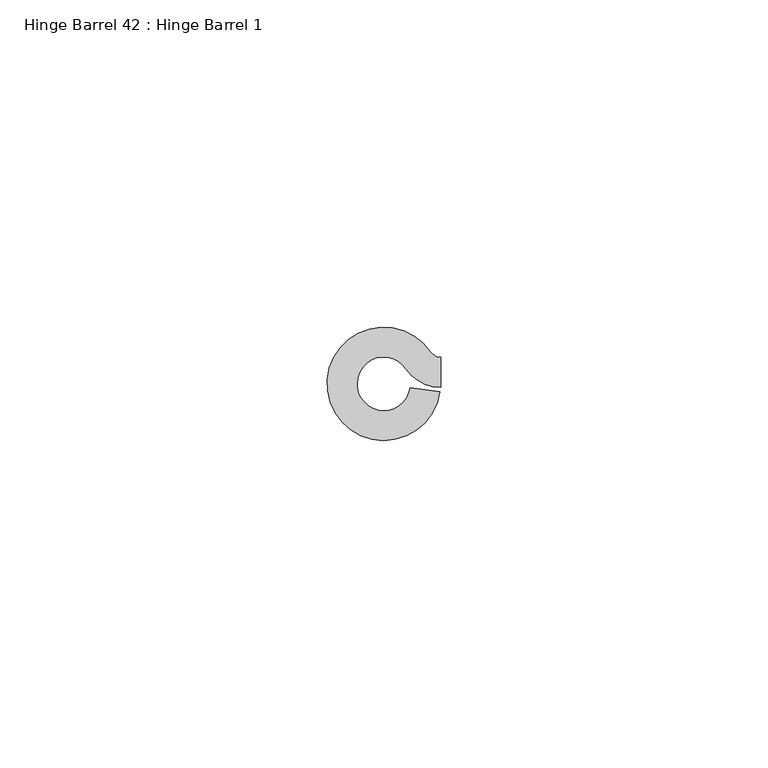
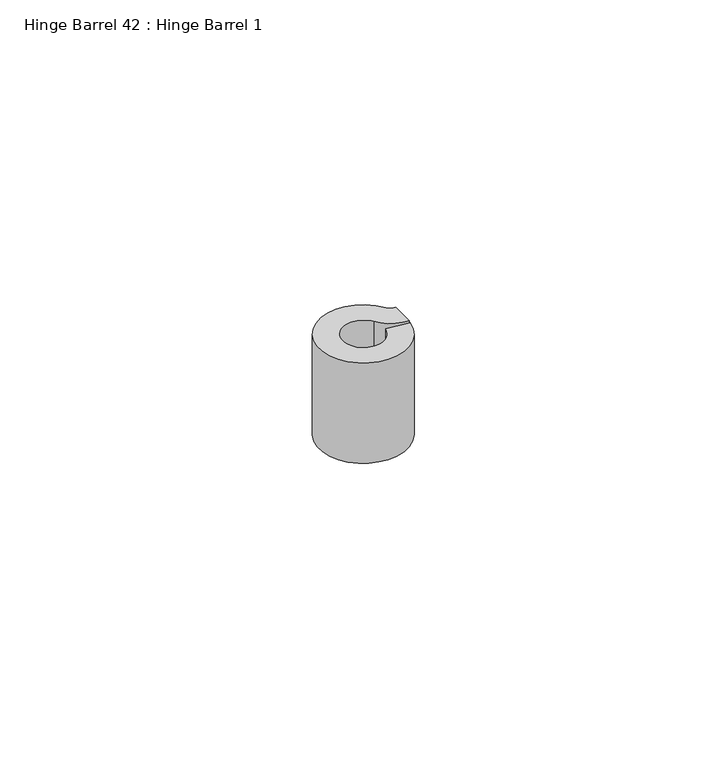
"""IFC4 building model written with IfcOpenShell, lengths in millimetres: proxy geometry, Hinge Barrel 42 : Hinge Barrel 1."""

import ifcopenshell
import ifcopenshell.guid

model = None  # the IFC model being written
_history = None  # IfcOwnerHistory: only IFC2X3 demands one
_inside = {}  # id of a spatial element -> (the spatial element, [elements in it])
_under = {}  # id of a project, library or spatial element -> (it, [spatial elements below it])
_declared = {}  # id of a project -> (the project, [libraries it declares])
_typed = {}  # id of a type object -> (the type object, [elements of that type])
_made_of = {}  # id of a material, layer set ... -> (it, [elements and type objects made of it])


def new_model(schema):
    """Start an empty IFC model of exactly this schema.

    Asked for "IFC4X3", IfcOpenShell would pick the latest addendum, in which some entities
    have other attributes; the version numbers below select the first issue.
    IFC2X3 requires an IfcOwnerHistory on every rooted entity: one is made here for all.
    """
    global model, _history
    if schema == "IFC4X3":
        model = ifcopenshell.file(schema_version=(4, 3, 0, 0))
    else:
        model = ifcopenshell.file(schema=schema)
    _inside.clear()
    _under.clear()
    _declared.clear()
    _typed.clear()
    _made_of.clear()
    _history = None
    if model.schema == "IFC2X3":
        org = make("IfcOrganization", Name="unknown")
        user = make(
            "IfcPersonAndOrganization",
            ThePerson=make("IfcPerson", FamilyName="unknown"),
            TheOrganization=org,
        )
        app = make(
            "IfcApplication",
            ApplicationDeveloper=org,
            Version="unknown",
            ApplicationFullName="unknown",
            ApplicationIdentifier="unknown",
        )
        _history = make(
            "IfcOwnerHistory",
            OwningUser=user,
            OwningApplication=app,
            ChangeAction="ADDED",
            CreationDate=0,
        )
    return model


def make(cls, **values):
    """One entity of the class cls with the attributes given. An attribute that is None is left unset."""
    return model.create_entity(
        cls, **{name: value for name, value in values.items() if value is not None}
    )


def rooted(cls, **values):
    """An entity with a GlobalId (a new one), such as an element, a storey or a relation."""
    return make(cls, GlobalId=ifcopenshell.guid.new(), OwnerHistory=_history, **values)


def si_unit(unit_type, name, prefix=None):
    """IfcSIUnit, for example si_unit("LENGTHUNIT", "METRE", prefix="MILLI")."""
    return make("IfcSIUnit", UnitType=unit_type, Prefix=prefix, Name=name)


def assignment(units):
    """IfcUnitAssignment: the units of a project."""
    return None if units is None else make("IfcUnitAssignment", Units=units)


def point(xyz):
    """IfcCartesianPoint."""
    return None if xyz is None else make("IfcCartesianPoint", Coordinates=xyz)


def direction(xyz):
    """IfcDirection."""
    return None if xyz is None else make("IfcDirection", DirectionRatios=xyz)


def frame(location, z_axis=None, x_axis=None):
    """IfcAxis2Placement3D, a coordinate frame: its origin and axes. An axis left out is left unset."""
    return make(
        "IfcAxis2Placement3D",
        Location=point(location),
        Axis=direction(z_axis),
        RefDirection=direction(x_axis),
    )


def frame_2d(location, x_axis=None):
    """IfcAxis2Placement2D, a coordinate frame in the plane: its origin and x axis."""
    return make(
        "IfcAxis2Placement2D", Location=point(location), RefDirection=direction(x_axis)
    )


def origin():
    """The frame at (0, 0, 0) with its axes left unset."""
    return frame((0.0, 0.0, 0.0))


def place(relative_to, where):
    """IfcLocalPlacement: puts the frame where relative to a parent placement (None: the world)."""
    return make(
        "IfcLocalPlacement", PlacementRelTo=relative_to, RelativePlacement=where
    )


def context(
    kind, dimensions, precision=None, world=None, true_north=None, identifier=None
):
    """IfcGeometricRepresentationContext, for example the 3D "Model" context."""
    return make(
        "IfcGeometricRepresentationContext",
        ContextIdentifier=identifier,
        ContextType=kind,
        CoordinateSpaceDimension=dimensions,
        Precision=precision,
        WorldCoordinateSystem=world,
        TrueNorth=true_north,
    )


def project(units=None, contexts=None):
    """IfcProject with its units and contexts."""
    return rooted(
        "IfcProject",
        Name="project",
        RepresentationContexts=contexts,
        UnitsInContext=assignment(units),
    )


def spatial(cls, under=None, at=None, **own):
    """A site, building, storey or space (cls), placed at a placement, below another one or the project."""
    s = rooted(cls, ObjectPlacement=at, **own)
    if under is not None:
        _under.setdefault(under.id(), (under, []))[1].append(s)
    return s


def polyline(points):
    """IfcPolyline through the points."""
    return make("IfcPolyline", Points=[point(p) for p in points])


def circle_curve(where, radius):
    """IfcCircle in the frame where."""
    return make("IfcCircle", Position=where, Radius=radius)


def trimmed(basis, trim1, trim2, sense, master):
    """IfcTrimmedCurve: the piece of a basis curve between two trims."""
    return make(
        "IfcTrimmedCurve",
        BasisCurve=basis,
        Trim1=trim1,
        Trim2=trim2,
        SenseAgreement=sense,
        MasterRepresentation=master,
    )


def segment(curve, same_sense, transition):
    """IfcCompositeCurveSegment."""
    return make(
        "IfcCompositeCurveSegment",
        Transition=transition,
        SameSense=same_sense,
        ParentCurve=curve,
    )


def composite_curve(segments, self_intersect=None):
    """IfcCompositeCurve: segments joined end to end."""
    return make("IfcCompositeCurve", Segments=segments, SelfIntersect=self_intersect)


def outline(outer, holes=None, kind="AREA"):
    """IfcArbitraryClosedProfileDef: a profile drawn as a closed curve; with holes, ...WithVoids."""
    if holes is None:
        return make("IfcArbitraryClosedProfileDef", ProfileType=kind, OuterCurve=outer)
    return make(
        "IfcArbitraryProfileDefWithVoids",
        ProfileType=kind,
        OuterCurve=outer,
        InnerCurves=holes,
    )


def extrude(swept, where, along, depth):
    """IfcExtrudedAreaSolid: the profile swept, set in the frame where, extruded along a direction by depth."""
    return make(
        "IfcExtrudedAreaSolid",
        SweptArea=swept,
        Position=where,
        ExtrudedDirection=direction(along),
        Depth=depth,
    )


def shape(context_of_items, identifier, shape_type, items):
    """IfcShapeRepresentation: the items that make up one representation, for example the "Body"."""
    return make(
        "IfcShapeRepresentation",
        ContextOfItems=context_of_items,
        RepresentationIdentifier=identifier,
        RepresentationType=shape_type,
        Items=items,
    )


def source(mapping_origin, context_of_items, identifier, shape_type, items):
    """IfcRepresentationMap: a shape defined once, which mapped items show again and again."""
    return make(
        "IfcRepresentationMap",
        MappingOrigin=mapping_origin,
        MappedRepresentation=shape(context_of_items, identifier, shape_type, items),
    )


def transform(
    local_origin,
    x_axis=None,
    y_axis=None,
    z_axis=None,
    scale=None,
    scale2=None,
    scale3=None,
    uniform=True,
):
    """IfcCartesianTransformationOperator3D, or its non-uniform kind. x_axis, y_axis, z_axis: its Axis1, 2, 3."""
    if uniform:
        return make(
            "IfcCartesianTransformationOperator3D",
            Axis1=direction(x_axis),
            Axis2=direction(y_axis),
            LocalOrigin=point(local_origin),
            Scale=scale,
            Axis3=direction(z_axis),
        )
    return make(
        "IfcCartesianTransformationOperator3DnonUniform",
        Axis1=direction(x_axis),
        Axis2=direction(y_axis),
        LocalOrigin=point(local_origin),
        Scale=scale,
        Axis3=direction(z_axis),
        Scale2=scale2,
        Scale3=scale3,
    )


def mapped(mapping_source, mapping_target):
    """IfcMappedItem: shows the shape of a source again, moved by a transform."""
    return make(
        "IfcMappedItem", MappingSource=mapping_source, MappingTarget=mapping_target
    )


def made_of(thing, what):
    """Note that an element or type object is made of a material, layer set ...; save() writes the relation."""
    if what is not None:
        _made_of.setdefault(what.id(), (what, []))[1].append(thing)
    return thing


def element(
    cls,
    number,
    at=None,
    inside=None,
    cuts=None,
    type_object=None,
    material=None,
    context=None,
    identifier="Body",
    shape_type=None,
    held_by="IfcProductDefinitionShape",
    body=None,
    shapes=None,
    **own,
):
    """One element of the class cls, such as IfcWall. Its Tag is "e" and its number.

    at: its placement. inside: the storey or other place that contains it. cuts: it is an
    opening in that element (IfcRelVoidsElement). A single representation is given by context,
    identifier, shape_type and body (its items); several are given by shapes. held_by: the class
    of the entity that holds the representations. save() writes the other relations.
    """
    e = rooted(cls, Tag="e%d" % number, ObjectPlacement=at, **own)
    if body is not None:
        shapes = [shape(context, identifier, shape_type, body)]
    if shapes is not None:
        e.Representation = make(held_by, Representations=shapes)
    if inside is not None:
        _inside.setdefault(inside.id(), (inside, []))[1].append(e)
    if cuts is not None:
        rooted(
            "IfcRelVoidsElement", RelatingBuildingElement=cuts, RelatedOpeningElement=e
        )
    if type_object is not None:
        _typed.setdefault(type_object.id(), (type_object, []))[1].append(e)
    return made_of(e, material)


def aggregate(whole, parts):
    """IfcRelAggregates: a whole, such as a stair, and the parts it consists of."""
    return rooted("IfcRelAggregates", RelatingObject=whole, RelatedObjects=parts)


def save(model, path):
    """Write the relations noted so far, then the file.

    IfcRelAggregates (storeys below a building ...), IfcRelContainedInSpatialStructure (elements
    in a storey), IfcRelDefinesByType, IfcRelAssociatesMaterial and IfcRelDeclares: one each for
    every whole, place, type object, material and project.
    """
    for whole, parts in _under.values():
        aggregate(whole, parts)
    for where, things in _inside.values():
        rooted(
            "IfcRelContainedInSpatialStructure",
            RelatedElements=things,
            RelatingStructure=where,
        )
    for kind, things in _typed.values():
        rooted("IfcRelDefinesByType", RelatedObjects=things, RelatingType=kind)
    for what, things in _made_of.values():
        rooted("IfcRelAssociatesMaterial", RelatedObjects=things, RelatingMaterial=what)
    for by, libraries in _declared.values():
        rooted("IfcRelDeclares", RelatingContext=by, RelatedDefinitions=libraries)
    model.write(path)


def hinge_barrel_42_hinge_barrel_1_1e33f8db(model_context):
    return source(origin(), model_context, "Body", "SweptSolid", [
        extrude(outline(composite_curve([segment(trimmed(circle_curve(frame_2d((587319.1320739, -534100.7049841)), 4.0894), [point((587322.5194669, -534098.4139665))], [point((587323.1821338, -534101.2708529))], True, "CARTESIAN"), True, "CONTINUOUS"), segment(polyline([(587323.1821338, -534101.2708529), (587327.7022899, -534101.9024028)]), True, "CONTINUOUS"), segment(trimmed(circle_curve(frame_2d((587319.1320739, -534100.7049841)), 8.6534625), [point((587327.7022899, -534101.9024028))], [point((587326.3000393, -534095.8570273))], False, "CARTESIAN"), True, "CONTINUOUS"), segment(trimmed(circle_curve(frame_2d((587327.8245257, -534094.8259615)), 1.8404226), [point((587326.3000393, -534095.8570273))], [point((587327.8245257, -534096.6663841))], True, "CARTESIAN"), True, "CONTINUOUS"), segment(polyline([(587327.8245257, -534096.6663841), (587327.8245257, -534101.2304466)]), True, "CONTINUOUS"), segment(trimmed(circle_curve(frame_2d((587327.8245257, -534094.8259615)), 6.4044851), [point((587327.8245257, -534101.2304466))], [point((587322.5194669, -534098.4139665))], False, "CARTESIAN"), True, "CONTINUOUS")], self_intersect=False)), frame((0.0, 0.0, 438.15), z_axis=(0.0, 0.0, 1.0), x_axis=(1.0, 0.0, 0.0)), (0.0, 0.0, 1.0), 20.8359375),
    ])


if __name__ == "__main__":
    model = new_model("IFC4")
    model_context = context("Model", 3, world=origin())
    ifc_project = project(units=[si_unit("LENGTHUNIT", "METRE", prefix="MILLI")], contexts=[model_context])
    site = spatial("IfcSite", under=ifc_project)
    building = spatial("IfcBuilding", under=site)
    placement = place(None, origin())
    hinge_barrel_42_hinge_barrel_1_shape = hinge_barrel_42_hinge_barrel_1_1e33f8db(model_context)
    element("IfcBuildingElementProxy", 1, Name="Hinge Barrel 42 : Hinge Barrel 1", ObjectType="Hinge Barrel 42 : Hinge Barrel 1", at=placement, inside=building, context=model_context, shape_type="MappedRepresentation", body=[
        mapped(hinge_barrel_42_hinge_barrel_1_shape, transform((0.0, 0.0, 0.0), x_axis=(1.0, 0.0, 0.0), y_axis=(0.0, 1.0, 0.0), z_axis=(0.0, 0.0, 1.0))),
    ])
    save(model, "model.ifc")

# Revit data of these elements
# Element 1 (IfcBuildingElementProxy, "Hinge Barrel 42 : Hinge Barrel 1")
#   Materials on its faces: "6\"X6\" WELD-ON STL BUTT HINGE"
# Materials
#   "6\"X6\" WELD-ON STL BUTT HINGE": class "Metal", colour RGB 189 187 185, transparency 0, Description = "Carbon steel", Cost = 0
